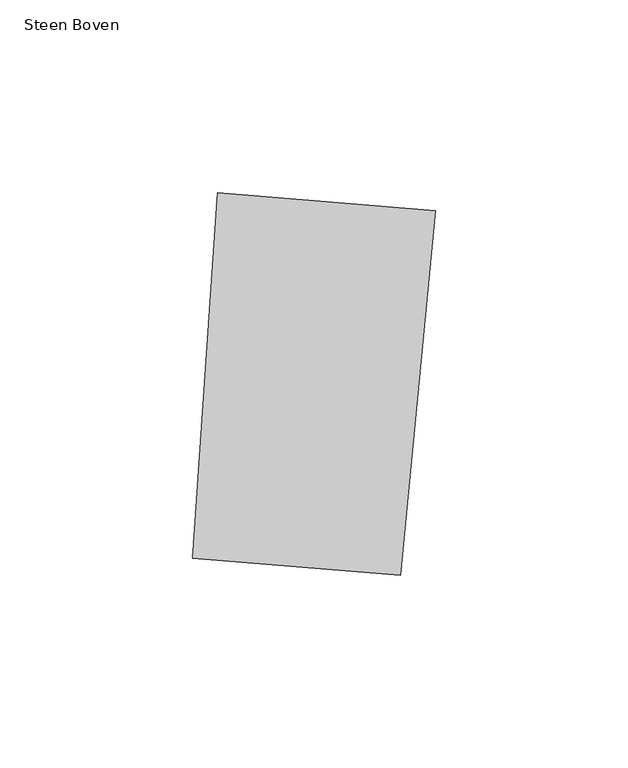
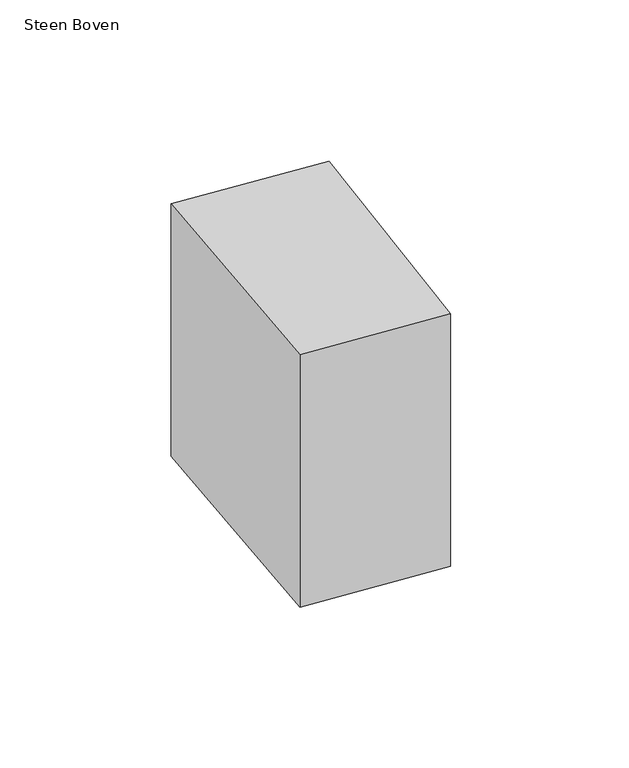
"""IFC4 building model written with IfcOpenShell, lengths in millimetres: proxy geometry, 00_GMA_steen_versie_4 : Steen Boven."""

from ifc_helpers import new_model, si_unit, origin, origin_with_axes, place, context, project, spatial, polyline, outline, extrude, source, transform, mapped, element, save


def steen_boven_4007128b(model_context):
    return source(origin(), model_context, "Body", "SweptSolid", [
        extrude(outline(polyline([(105.324489, 118.7832041), (96.2907047, 24.2047729), (42.3388117, 28.6330613), (48.8477413, 123.4187286), (105.324489, 118.7832041)])), origin_with_axes(), (0.0, 0.0, 1.0), 100.0),
    ])


if __name__ == "__main__":
    model = new_model("IFC4")
    model_context = context("Model", 3, world=origin())
    ifc_project = project(units=[si_unit("LENGTHUNIT", "METRE", prefix="MILLI")], contexts=[model_context])
    site = spatial("IfcSite", under=ifc_project)
    building = spatial("IfcBuilding", under=site)
    placement = place(None, origin())
    steen_boven_shape = steen_boven_4007128b(model_context)
    element("IfcBuildingElementProxy", 1, Name="00_GMA_steen_versie_4 : Steen Boven", ObjectType="00_GMA_steen_versie_4 : Steen Boven", at=placement, inside=building, context=model_context, shape_type="MappedRepresentation", body=[
        mapped(steen_boven_shape, transform((0.0, 0.0, 0.0), x_axis=(1.0, 0.0, 0.0), y_axis=(0.0, 1.0, 0.0), z_axis=(0.0, 0.0, 1.0))),
    ])
    save(model, "model.ifc")

# Revit data of these elements
# Type "00_GMA_steen_versie_4 : Steen Boven"
#   StootVoegHalfBoven [instance default] = 5 mm
#   StootVoegHalf [instance default] = 5 mm
#   StootVoegBreedteOnder = 10 mm
#   StootVoegBreedteBoven = 10 mm
#   Steendikte = 100 mm
#   LintVoegOnderHalf = 5 mm
#   LintVoegOnder = 10 mm
#   LintVoegBovenHalf = 0 mm
#   LintVoegBoven = 0 mm
#   materiaal = none
#   MateriaalVoeg = none
#   Default Elevation = 0
